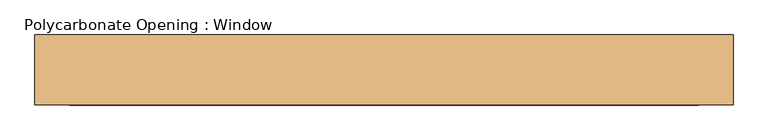
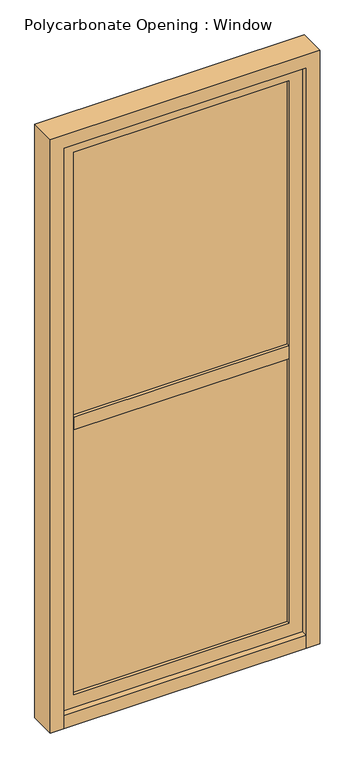
"""IFC4 building model written with IfcOpenShell, lengths in millimetres: door geometry, Polycarbonate Opening : Window."""

from ifc_helpers import new_model, si_unit, frame, origin, origin_with_axes, place, context, project, spatial, polyline, outline, extrude, source, transform, mapped, element, save


def polycarbonate_opening_window_95fe8ec7(model_context):
    return source(origin(), model_context, "Body", "SweptSolid", [
        extrude(outline(polyline([(457.2, 12.7), (457.2, -12.7), (-457.2, -12.7), (-457.2, 12.7), (457.2, 12.7)])), frame((0.0, 0.0, 50.8), z_axis=(0.0, 0.0, 1.0), x_axis=(1.0, 0.0, 0.0)), (0.0, 0.0, 1.0), 2260.6),
        extrude(outline(polyline([(2311.4, -457.2), (0.0, -457.2), (0.0, 457.2), (2311.4, 457.2), (2311.4, -457.2)]), holes=[polyline([(101.6, 406.4), (101.6, -406.4), (2260.6, -406.4), (2260.6, 406.4), (101.6, 406.4)])]), frame((0.0, -25.4, 0.0), z_axis=(0.0, 1.0, 0.0), x_axis=(0.0, 0.0, 1.0)), (0.0, 0.0, 1.0), 50.8),
        extrude(outline(polyline([(2362.2, 508.0), (2362.2, -508.0), (0.0, -508.0), (0.0, -457.2), (2311.4, -457.2), (2311.4, 457.2), (0.0, 457.2), (0.0, 508.0), (2362.2, 508.0)])), frame((0.0, -50.8, 0.0), z_axis=(0.0, 1.0, 0.0), x_axis=(0.0, 0.0, 1.0)), (0.0, 0.0, 1.0), 101.6),
        extrude(outline(polyline([(406.4, 25.4), (406.4, -25.4), (-406.4, -25.4), (-406.4, 25.4), (406.4, 25.4)])), frame((0.0, 0.0, 1155.7), z_axis=(0.0, 0.0, 1.0), x_axis=(1.0, 0.0, 0.0)), (0.0, 0.0, 1.0), 50.8),
        extrude(outline(polyline([(457.2, 50.8), (457.2, -50.8), (-457.2, -50.8), (-457.2, 50.8), (457.2, 50.8)])), origin_with_axes(), (0.0, 0.0, 1.0), 50.8),
    ])


if __name__ == "__main__":
    model = new_model("IFC4")
    model_context = context("Model", 3, world=origin())
    ifc_project = project(units=[si_unit("LENGTHUNIT", "METRE", prefix="MILLI")], contexts=[model_context])
    site = spatial("IfcSite", under=ifc_project)
    building = spatial("IfcBuilding", under=site)
    placement = place(None, origin())
    polycarbonate_opening_window_shape = polycarbonate_opening_window_95fe8ec7(model_context)
    element("IfcDoor", 1, ObjectType="Polycarbonate Opening : Window", at=placement, inside=building, context=model_context, shape_type="MappedRepresentation", body=[
        mapped(polycarbonate_opening_window_shape, transform((0.0, 0.0, 0.0), x_axis=(1.0, 0.0, 0.0), y_axis=(0.0, 1.0, 0.0), z_axis=(0.0, 0.0, 1.0))),
    ])
    save(model, "model.ifc")

# Revit data of these elements
# Type "Polycarbonate Opening : Window"
#   Type Mark = "59"
#   Analytic Construction = "<None>"
#   offset [instance default] = 0' - 2"
#   Stile = 0' - 2"
#   Mullion Width = 0' - 2"
#   Mullion Depth = 0' - 4"
#   Opening Size [instance default] = 5' - 1.50212"
#   Door Width [instance default] = 5' - 1.50212"
#   Window ON/OFF = no
#   Door On/Off = yes
#   Mullion Material = ALUMINUM STOREFRONT
#   Glass Material = INSULATED GLAZING
#   Door Material = ALUMINUM STOREFRONT
# Element 1 (IfcDoor, "Polycarbonate Opening : Window")
#   offset = 0' - 0"
#   Materials on its faces: "ALUMINUM STOREFRONT", "INSULATED GLAZING"
# Materials
#   "ALUMINUM STOREFRONT": class "Metal", colour RGB 244 244 244, transparency 0, Description = "Aluminum 6061", Cost = 0
#   "INSULATED GLAZING": class "Glass", colour RGB 196 205 210, transparency 0.85, Description = "Soda Lime Glass", Cost = 0
